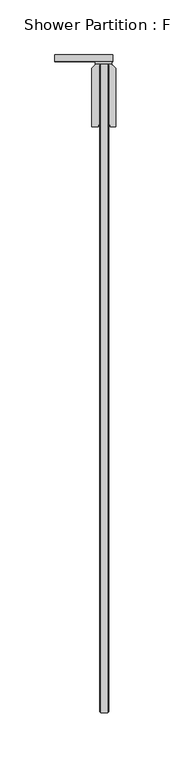
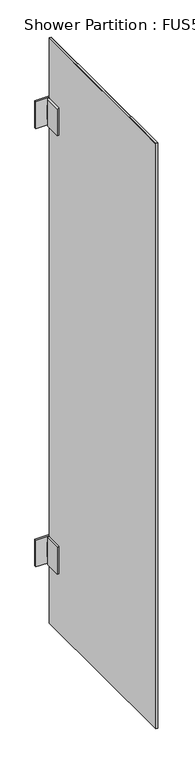
"""IFC4 building model written with IfcOpenShell, lengths in millimetres: furniture geometry, Shower Partition : FUS501_Shower Partition."""

from ifc_helpers import new_model, si_unit, origin, place, context, project, spatial, faceted_brep, source, transform, mapped, element, save


def shower_partition_fus501_shower_partition_1146f189(model_context):
    return source(origin(), model_context, "Body", "Brep", [
        faceted_brep([(17.0, 294.0, 1761.208438), (2.0, 294.0, 1761.208438), (2.0, 291.5, 1761.208438), (6.9579486, 291.5, 1761.208438), (13.0420514, 291.5, 1761.208438), (17.0, 291.5, 1761.208438), (2.0, 291.5, 1785.5), (6.9579486, 291.5, 1785.5), (13.0420514, 291.5, 1785.5), (17.0, 291.5, 1785.5), (2.0, 291.5, 1713.920216), (6.9579486, 291.5, 1713.920216), (6.9579486, 291.5, 1694.5), (2.0, 291.5, 1694.5), (13.0420514, 291.5, 1713.920216), (17.0, 291.5, 1713.920216), (17.0, 291.5, 1694.5), (13.0420514, 291.5, 1694.5), (2.0, 294.0, 1713.920216), (17.0, 294.0, 1713.920216), (2.0, 290.5420514, 1785.5), (1.2131065, 290.5420514, 1785.5), (-1.5, 287.828945, 1785.5), (-1.5, 234.5, 1785.5), (4.5, 234.5, 1785.5), (4.5, 236.5, 1785.5), (6.0, 236.5, 1785.5), (6.0, 290.5420514, 1785.5), (14.0, 290.5420514, 1785.5), (14.0, 236.5, 1785.5), (15.5, 236.5, 1785.5), (15.5, 234.5, 1785.5), (20.5, 234.5, 1785.5), (20.5, 287.828945, 1785.5), (17.7868935, 290.5420514, 1785.5), (17.0, 290.5420514, 1785.5), (-35.0, 294.0, 1785.5), (17.8567847, 294.0, 1785.5), (17.8567847, 300.0, 1785.5), (-35.0, 300.0, 1785.5), (17.0, 290.5420514, 1694.5), (17.7868935, 290.5420514, 1694.5), (20.5, 287.828945, 1694.5), (20.5, 234.5, 1694.5), (15.5, 234.5, 1694.5), (15.5, 236.5, 1694.5), (14.0, 236.5, 1694.5), (14.0, 290.5420514, 1694.5), (6.0, 290.5420514, 1694.5), (6.0, 236.5, 1694.5), (4.5, 236.5, 1694.5), (4.5, 234.5, 1694.5), (-1.5, 234.5, 1694.5), (-1.5, 287.828945, 1694.5), (1.2131065, 290.5420514, 1694.5), (2.0, 290.5420514, 1694.5), (17.8567847, 294.0, 1694.5), (-35.0, 294.0, 1694.5), (-35.0, 300.0, 1694.5), (17.8567847, 300.0, 1694.5)], [[[0, 1, 2, 3, 4, 5]], [[3, 2, 6, 7]], [[5, 4, 8, 9]], [[10, 11, 12, 13]], [[14, 15, 16, 17]], [[18, 19, 15, 14, 11, 10]], [[20, 21, 22, 23, 24, 25, 26, 27, 7, 6]], [[8, 28, 29, 30, 31, 32, 33, 34, 35, 9]], [[36, 37, 38, 39]], [[40, 41, 42, 43, 44, 45, 46, 47, 17, 16]], [[12, 48, 49, 50, 51, 52, 53, 54, 55, 13]], [[56, 57, 58, 59]], [[36, 57, 56, 37], [1, 0, 19, 18]], [[55, 20, 6, 2, 1, 18, 10, 13]], [[21, 20, 55, 54]], [[22, 21, 54, 53]], [[23, 22, 53, 52]], [[24, 23, 52, 51]], [[25, 24, 51, 50]], [[29, 28, 47, 46]], [[30, 29, 46, 45]], [[31, 30, 45, 44]], [[32, 31, 44, 43]], [[33, 32, 43, 42]], [[34, 33, 42, 41]], [[35, 34, 41, 40]], [[35, 40, 16, 15, 19, 0, 5, 9]], [[38, 37, 56, 59]], [[39, 38, 59, 58]], [[36, 39, 58, 57]], [[26, 25, 50, 49]], [[27, 26, 49, 48]], [[7, 27, 48, 12, 11, 3]], [[3, 11, 14, 4]], [[28, 8, 4, 14, 17, 47]]]),
        faceted_brep([(2.0, 290.5420514, 295.5), (1.2131065, 290.5420514, 295.5), (-1.5, 287.828945, 295.5), (-1.5, 234.5, 295.5), (4.5, 234.5, 295.5), (4.5, 236.5, 295.5), (6.0, 236.5, 295.5), (6.0, 290.5420514, 295.5), (6.9579486, 291.5, 295.5), (2.0, 291.5, 295.5), (13.0420514, 291.5, 295.5), (14.0, 290.5420514, 295.5), (14.0, 236.5, 295.5), (15.5, 236.5, 295.5), (15.5, 234.5, 295.5), (20.5, 234.5, 295.5), (20.5, 287.828945, 295.5), (17.7868935, 290.5420514, 295.5), (17.0, 290.5420514, 295.5), (17.0, 291.5, 295.5), (-35.0, 294.0, 295.5), (17.8567847, 294.0, 295.5), (17.8567847, 300.0, 295.5), (-35.0, 300.0, 295.5), (17.0, 290.5420514, 204.5), (17.7868935, 290.5420514, 204.5), (20.5, 287.828945, 204.5), (20.5, 234.5, 204.5), (15.5, 234.5, 204.5), (15.5, 236.5, 204.5), (14.0, 236.5, 204.5), (14.0, 290.5420514, 204.5), (13.0420514, 291.5, 204.5), (17.0, 291.5, 204.5), (6.9579486, 291.5, 204.5), (6.0, 290.5420514, 204.5), (6.0, 236.5, 204.5), (4.5, 236.5, 204.5), (4.5, 234.5, 204.5), (-1.5, 234.5, 204.5), (-1.5, 287.828945, 204.5), (1.2131065, 290.5420514, 204.5), (2.0, 290.5420514, 204.5), (2.0, 291.5, 204.5), (17.8567847, 294.0, 204.5), (-35.0, 294.0, 204.5), (-35.0, 300.0, 204.5), (17.8567847, 300.0, 204.5), (2.0, 294.0, 276.079784), (17.0, 294.0, 276.079784), (17.0, 294.0, 226.670216), (2.0, 294.0, 226.670216), (2.0, 291.5, 276.079784), (2.0, 291.5, 226.670216), (17.0, 291.5, 226.670216), (17.0, 291.5, 276.079784), (6.9579486, 291.5, 276.079784), (13.0420514, 291.5, 276.079784), (6.9579486, 291.5, 226.670216), (13.0420514, 291.5, 226.670216)], [[[0, 1, 2, 3, 4, 5, 6, 7, 8, 9]], [[10, 11, 12, 13, 14, 15, 16, 17, 18, 19]], [[20, 21, 22, 23]], [[24, 25, 26, 27, 28, 29, 30, 31, 32, 33]], [[34, 35, 36, 37, 38, 39, 40, 41, 42, 43]], [[44, 45, 46, 47]], [[20, 45, 44, 21], [48, 49, 50, 51]], [[42, 0, 9, 52, 48, 51, 53, 43]], [[1, 0, 42, 41]], [[2, 1, 41, 40]], [[3, 2, 40, 39]], [[4, 3, 39, 38]], [[5, 4, 38, 37]], [[12, 11, 31, 30]], [[13, 12, 30, 29]], [[14, 13, 29, 28]], [[15, 14, 28, 27]], [[16, 15, 27, 26]], [[17, 16, 26, 25]], [[18, 17, 25, 24]], [[18, 24, 33, 54, 50, 49, 55, 19]], [[22, 21, 44, 47]], [[23, 22, 47, 46]], [[20, 23, 46, 45]], [[49, 48, 52, 56, 57, 55]], [[56, 52, 9, 8]], [[55, 57, 10, 19]], [[53, 58, 34, 43]], [[59, 54, 33, 32]], [[51, 50, 54, 59, 58, 53]], [[6, 5, 37, 36]], [[7, 6, 36, 35]], [[8, 7, 35, 34, 58, 56]], [[56, 58, 59, 57]], [[11, 10, 57, 59, 32, 31]]]),
        faceted_brep([(13.0420514, -300.0, 0.0), (6.9579486, -300.0, 0.0), (6.9579486, 291.5, 0.0), (13.0420514, 291.5, 0.0), (13.0420514, 291.5, 1990.0), (6.9579486, 291.5, 1990.0), (6.9579486, -300.0, 1990.0), (13.0420514, -300.0, 1990.0), (6.0, -299.0420514, 0.9579486), (6.0, -299.0420514, 1989.0420514), (6.0, 290.5420514, 1989.0420514), (6.0, 290.5420514, 0.9579486), (14.0, -299.0420514, 1989.0420514), (14.0, -299.0420514, 0.9579486), (14.0, 290.5420514, 0.9579486), (14.0, 290.5420514, 1989.0420514)], [[[0, 1, 2, 3]], [[4, 5, 6, 7]], [[1, 0, 7, 6]], [[8, 9, 10, 11]], [[3, 2, 5, 4]], [[12, 13, 14, 15]], [[8, 1, 6, 9]], [[1, 8, 11, 2]], [[2, 11, 10, 5]], [[9, 6, 5, 10]], [[0, 13, 12, 7]], [[13, 0, 3, 14]], [[14, 3, 4, 15]], [[7, 12, 15, 4]]]),
    ])


if __name__ == "__main__":
    model = new_model("IFC4")
    model_context = context("Model", 3, world=origin())
    ifc_project = project(units=[si_unit("LENGTHUNIT", "METRE", prefix="MILLI")], contexts=[model_context])
    site = spatial("IfcSite", under=ifc_project)
    building = spatial("IfcBuilding", under=site)
    placement = place(None, origin())
    shower_partition_fus501_shower_partition_shape = shower_partition_fus501_shower_partition_1146f189(model_context)
    element("IfcFurniture", 1, ObjectType="Shower Partition : FUS501_Shower Partition", at=placement, inside=building, context=model_context, shape_type="MappedRepresentation", body=[
        mapped(shower_partition_fus501_shower_partition_shape, transform((0.0, 0.0, 0.0), x_axis=(1.0, 0.0, 0.0), y_axis=(0.0, 1.0, 0.0), z_axis=(0.0, 0.0, 1.0))),
    ])
    save(model, "model.ifc")

# Revit data of these elements
# Type "Shower Partition : FUS501_Shower Partition"
#   Youtube clip = ""
#   Weight Net (Kg) = "0"
#   Weight = ""
#   WarrantyStartDate [instance default] = "n/a"
#   WarrantyGuarantorParts = "n/a"
#   WarrantyGuarantorLabor = "n/a"
#   WarrantyDurationUnit = "Year"
#   WarrantyDurationParts = "n/a"
#   WarrantyDurationLabor = "n/a"
#   WarrantyDescription = "n/a"
#   VersionDate = "03/02/2020"
#   Version = "1"
#   Uniformat II Description = ""
#   Uniformat II Code = ""
#   Uniclass2015Reference = "Pr_40_20_06_79"
#   Uniclass2015Description = "Shower enclosures"
#   Uniclass2 = "Pr_40_30_06_79"
#   Uniclass 2015 Name = ""
#   Uniclass 2015 Code = ""
#   Uniclass 2.0 Description = ""
#   Uniclass 2.0 Code = ""
#   Uniclass 1.4 Description = ""
#   Uniclass 1.4 Code = ""
#   URL = "https://www.svedbergs.com/products/showers/shower-screen/180-shower-screen-1-door-78-206348/"
#   UNSPSC Code = ""
#   Technical description = ""
#   TagNumber [instance default] = "n/a"
#   SustainabilityPerformance = "n/a"
#   Style = "n/a"
#   Size = "70x780x2000mm"
#   Shape = "Rectangular"
#   SerialNumber [instance default] = "n/a"
#   Revision = "n/a"
#   ReplacementCost = "n/a"
#   Region South America = "All"
#   Region Oceania = "All"
#   Region North America = "All"
#   Region Middle East = "All"
#   Region Europe = "All"
#   Region Asia = "All"
#   Region Antarctica = "All"
#   Region Africa = "All"
#   RSKNumber = "7331415"
#   QR code = "http://bimobject.com/svedbergs/product/shower-78_shower"
#   ProductInformation = "Has one opening door. Doors can be folded inwards when shower is not in use to maximise floor space. No threshold – allows disabled access. Toughened safety glass 8 mm. Self-closing hinges. Concealed mounting & clamping screws. Height 200 cm. Door opening 75-95 cm."
#   ProductDatasheet = "https://www.svedbergs.com/products/showers/shower-screen/180-shower-screen-1-door-78-206348/GetPdf/?code=206348&productName=180%C2%B0%20Shower%20screen%201%20door%2078"
#   Product url = "https://www.svedbergs.com/products/showers/shower-screen/180-shower-screen-1-door-78-206348/"
#   Product group = "Shower Screen"
#   Product family = "180"
#   Product data url = "https://bimobject.com/svedbergs/product/shower-78_shower"
#   Product certification = ""
#   Product SKU = "shower-78_shower"
#   Product Guid = "bad75198-8fba-4d63-8e5f-588e794387c3"
#   OmniClass Description = ""
#   OmniClass Code = ""
#   Name = "180_Shower-screen_78"
#   NBSReference = "45-35-70/332"
#   NBSDescription = "Shower enclosures"
#   NBS Reference Description = ""
#   NBS Reference Code = ""
#   ModelReference = "681778"
#   ModelNumber = "n/a"
#   Material secondary = ""
#   Material main = ""
#   Material = "Glass, metal"
#   Masterformat 2014 Description = ""
#   Masterformat 2014 Code = ""
#   ManufacturerURL = "https://www.svedbergs.com/"
#   ManufacturerName = "Svedbergs"
#   Manufacturer name = ""
#   Manufacturer country = "Sweden"
#   MainColor = "Transparent"
#   InstallationDate [instance default] = "n/a"
#   Installation instructions = ""
#   IFC Classification = ""
#   GTIN code = ""
#   EANNumber = "7323100206787"
#   Design country = "Sweden"
#   Description = "Has one opening door. Doors can be folded inwards when shower is not in use to maximise floor space. No threshold – allows disabled access. Toughened safety glass 8 mm. Self-closing hinges. Concealed mounting & clamping screws. Height 200 cm. Door opening 75-95 cm."
#   Date of publishing = ""
#   Collection = "180°"
#   Model = "180° Shower Door 78 - Chrome/Clear glass"
#   Manufacturer = "Svedbergs"
#   IfcExportType = "NOTDEFINED"
#   IfcExportAs = "IfcFurnitureType"
#   Grade = "n/a"
#   Finish = "Black Mat/Clear glass"
#   Features = "Accessories:Shower seat Relax"
#   ExpectedLife = "n/a"
#   DurationUnit = "Year"
#   ConvergoRefNr = "0056-1912-0096-SE\t\t\r\n"
#   Constituents = "n/a"
#   Color = "Transparent"
#   CodePerformance = "n/a"
#   Category = "Shower screen"
#   COBIe Type Category = ""
#   Brand url = "http://www.svedbergs.com/"
#   Brand = "Svedbergs"
#   Barcode [instance default] = "n/a"
#   BIMobject main category code = "sanitary"
#   BIMobject main category = "Sanitary"
#   BIMobject category code = "sanitary-shower-screens"
#   BIMobject category = "Shower screens"
#   BIMObjectName = "Sanitary_Shower-screens_Svedbergs_180_Shower-screen_78"
#   Author = "Convergo AB"
#   AssetType = "Fixed"
#   AssetIdentifier [instance default] = "n/a"
#   AssemblyInstruction = "https://www.svedbergs.com/globalassets/catalog-assets/documentfile/99248-M1_180_dorr.pdf"
#   AccessibilityPerformance = "n/a"
#   NominalLength = 70 mm
#   NominalDepth = 600 mm
#   Nominal width = 0 mm
#   Nominal height = 0 mm
#   Edition number = 1
#   ShowerEnclosureSecondaryMaterial = Black Mat
#   ShowerEnclosureMainMaterial = Clear Glass
#   Type Comments = ""
#   Default Elevation = 0
#   Cost = 0
# Element 1 (IfcFurniture, "Shower Partition : FUS501_Shower Partition")
#   Materials on its faces: "Black Mat", "Clear Glass"
# Materials
#   "Black Mat": class "Metal", colour RGB 20 20 20, transparency 0, Cost = 0
#   "Clear Glass": class "Glass", colour RGB 236 240 239, transparency 0.85, Description = "Clear glazing", Cost = 0
